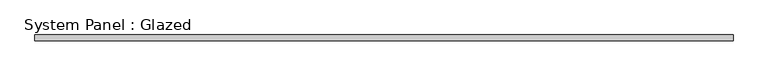
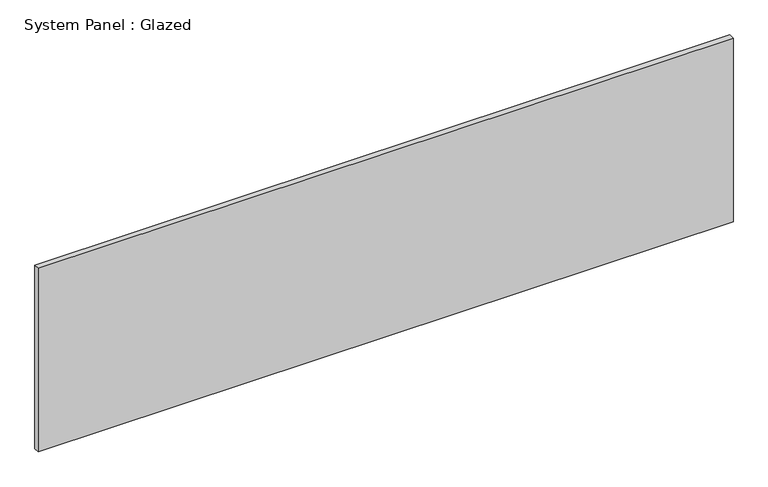
"""IFC4 building model written with IfcOpenShell, lengths in millimetres: plate geometry, System Panel : Glazed."""

from ifc_helpers import new_model, si_unit, origin, origin_with_axes, place, context, project, spatial, polyline, outline, extrude, source, transform, mapped, element, save


def system_panel_glazed_8bf11259(model_context):
    return source(origin(), model_context, "Body", "SweptSolid", [
        extrude(outline(polyline([(1549.4, -44.45), (-1549.4, -44.45), (-1549.4, -19.05), (1549.4, -19.05), (1549.4, -44.45)])), origin_with_axes(), (0.0, 0.0, 1.0), 866.0018549),
    ])


if __name__ == "__main__":
    model = new_model("IFC4")
    model_context = context("Model", 3, world=origin())
    ifc_project = project(units=[si_unit("LENGTHUNIT", "METRE", prefix="MILLI")], contexts=[model_context])
    site = spatial("IfcSite", under=ifc_project)
    building = spatial("IfcBuilding", under=site)
    placement = place(None, origin())
    system_panel_glazed_shape = system_panel_glazed_8bf11259(model_context)
    element("IfcPlate", 1, ObjectType="System Panel : Glazed", at=placement, inside=building, context=model_context, shape_type="MappedRepresentation", body=[
        mapped(system_panel_glazed_shape, transform((0.0, 0.0, 0.0), x_axis=(1.0, 0.0, 0.0), y_axis=(0.0, 1.0, 0.0), z_axis=(0.0, 0.0, 1.0))),
    ])
    save(model, "model.ifc")

# Revit data of these elements
# Type "System Panel : Glazed"
#   Construction Type Id = "GSP4R"
#   Analytic Construction = "1/8 in Pilkington single glazing"
#   Visual Light Transmittance = 0.9
#   Solar Heat Gain Coefficient = 0.86
#   Heat Transfer Coefficient (U) = 1.18115 BTU/(h·ft²·°F)
#   Define Thermal Properties by = 1
# Element 1 (IfcPlate, "System Panel : Glazed")
#   Materials on its faces: "Glass"
# Materials
#   "Glass": class "Glass", colour RGB 0 128 192, transparency 0.75, Description = "Soda Lime Glass", Cost = 0
